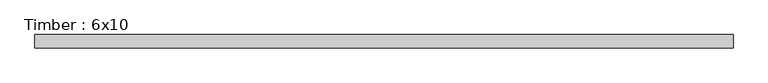
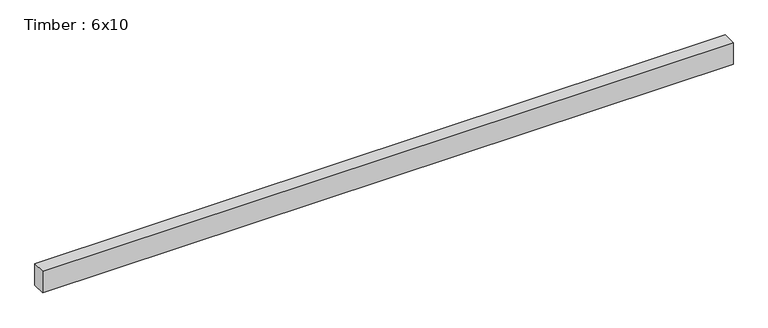
"""IFC4 building model written with IfcOpenShell, lengths in millimetres: beam geometry, Timber : 6x10."""

from ifc_helpers import new_model, si_unit, frame, origin, place, context, project, spatial, polyline, outline, extrude, source, transform, mapped, element, save


def timber_6x10_01175893(model_context):
    return source(origin(), model_context, "Body", "SweptSolid", [
        extrude(outline(polyline([(1821.0853, 69.85), (1821.0853, -69.85), (-5454.65, -69.85), (-5454.65, 69.85), (1821.0853, 69.85)])), frame((0.0, 0.0, -120.65), z_axis=(0.0, 0.0, 1.0), x_axis=(1.0, 0.0, 0.0)), (0.0, 0.0, 1.0), 241.3),
    ])


if __name__ == "__main__":
    model = new_model("IFC4")
    model_context = context("Model", 3, world=origin())
    ifc_project = project(units=[si_unit("LENGTHUNIT", "METRE", prefix="MILLI")], contexts=[model_context])
    site = spatial("IfcSite", under=ifc_project)
    building = spatial("IfcBuilding", under=site)
    placement = place(None, origin())
    timber_6x10_shape = timber_6x10_01175893(model_context)
    element("IfcBeam", 1, ObjectType="Timber : 6x10", at=placement, inside=building, context=model_context, shape_type="MappedRepresentation", body=[
        mapped(timber_6x10_shape, transform((0.0, 0.0, 0.0), x_axis=(1.0, 0.0, 0.0), y_axis=(0.0, 1.0, 0.0), z_axis=(0.0, 0.0, 1.0))),
    ])
    save(model, "model.ifc")

# Revit data of these elements
# Type "Timber : 6x10"
#   Assembly Code = "B10"
#   A = 0.362847 SF
#   Length [instance default] = 5' - 0"
#   b = 0' - 5 1/2"
#   d = 0' - 9 1/2"
#   Structural Material [instance default] = Softwood, Lumber
# Element 1 (IfcBeam, "Timber : 6x10")
#   Materials on its faces: "Softwood, Lumber"
# Materials
#   "Softwood, Lumber": class "Wood", colour RGB 144 113 62, transparency 0, Description = "Pinus Echinata", Cost = 0
